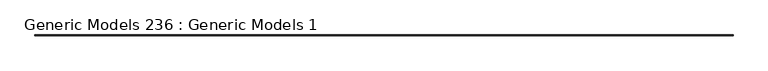
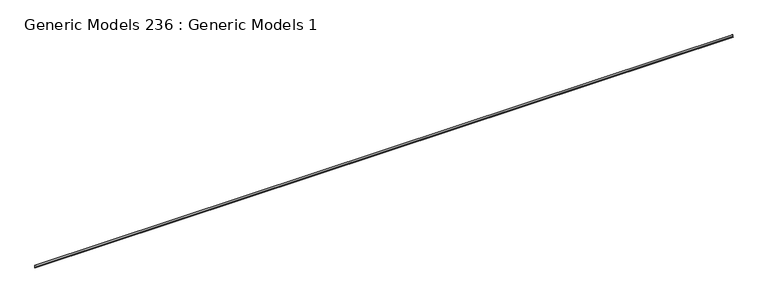
"""IFC4 building model written with IfcOpenShell, lengths in millimetres: proxy geometry, Generic Models 236 : Generic Models 1."""

from ifc_helpers import new_model, si_unit, frame, origin, place, context, project, spatial, polyline, outline, extrude, source, transform, mapped, element, save


def generic_models_236_generic_models_1_a805a110(model_context):
    return source(origin(), model_context, "Body", "SweptSolid", [
        extrude(outline(polyline([(-29389.2485041, 126996.7728942), (-29368.2935041, 127003.50843), (-29368.2935041, 127047.5728942), (-29367.0235041, 127047.5728942), (-29367.0235041, 127002.5826506), (-29385.0983018, 126996.7728942), (-29367.9866992, 126991.2727363), (-29367.0235041, 126986.1579859), (-29368.2715667, 126985.9229543), (-29369.0948876, 126990.2949461), (-29389.2485041, 126996.7728942)])), frame((-20998.9733045, 0.0, 0.0), z_axis=(1.0, 0.0, 0.0), x_axis=(0.0, 1.0, 0.0)), (0.0, 0.0, 1.0), 19050.0),
    ])


if __name__ == "__main__":
    model = new_model("IFC4")
    model_context = context("Model", 3, world=origin())
    ifc_project = project(units=[si_unit("LENGTHUNIT", "METRE", prefix="MILLI")], contexts=[model_context])
    site = spatial("IfcSite", under=ifc_project)
    building = spatial("IfcBuilding", under=site)
    placement = place(None, origin())
    generic_models_236_generic_models_1_shape = generic_models_236_generic_models_1_a805a110(model_context)
    element("IfcBuildingElementProxy", 1, Name="Generic Models 236 : Generic Models 1", ObjectType="Generic Models 236 : Generic Models 1", at=placement, inside=building, context=model_context, shape_type="MappedRepresentation", body=[
        mapped(generic_models_236_generic_models_1_shape, transform((0.0, 0.0, 0.0), x_axis=(1.0, 0.0, 0.0), y_axis=(0.0, 1.0, 0.0), z_axis=(0.0, 0.0, 1.0))),
    ])
    save(model, "model.ifc")

# Revit data of these elements
# Element 1 (IfcBuildingElementProxy, "Generic Models 236 : Generic Models 1")
#   Materials on its faces: "_16 GA. COPPER WEEP SCREED W/ MIN. 3 1/2\" ATTACHEMENT FLANGE - LAP UNDERLAYMENT OVER WEED SCREED"
# Materials
#   "_16 GA. COPPER WEEP SCREED W/ MIN. 3 1/2\" ATTACHEMENT FLANGE - LAP UNDERLAYMENT OVER WEED SCREED": class "Generic", colour RGB 253 192 103, transparency 0, Cost = 0
